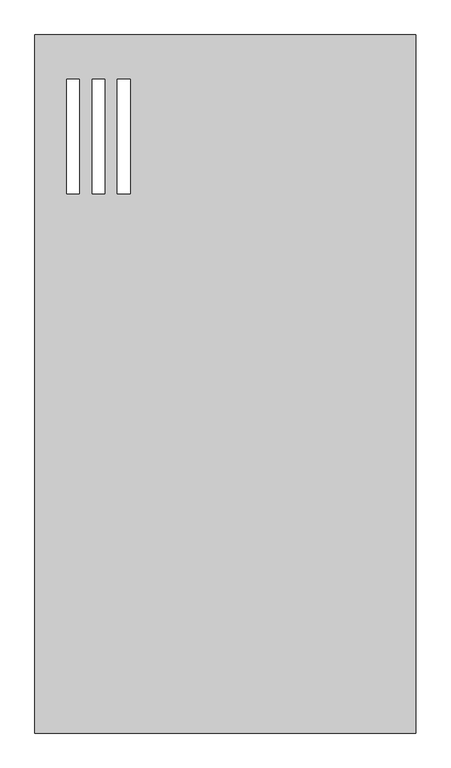
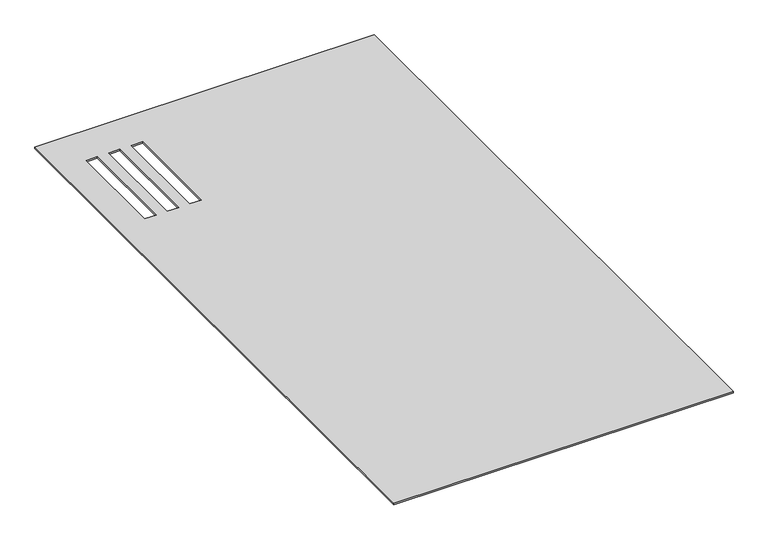
"""IFC4 building model written with IfcOpenShell, lengths in millimetres: proxy geometry, TSP Geyser Electrcical 300L : TSP Geyser Electrcical 300L."""

from ifc_helpers import new_model, si_unit, origin, origin_with_axes, place, context, project, spatial, polyline, outline, extrude, source, transform, mapped, element, save


def electrical_fixtures_aa66fa3b(model_context):
    return source(origin(), model_context, "Body", "SweptSolid", [
        extrude(outline(polyline([(-600.0, 600.0), (0.0, 600.0), (0.0, -500.0), (-600.0, -500.0), (-600.0, 600.0)]), holes=[polyline([(-530.0, 530.0), (-550.0, 530.0), (-550.0, 350.0), (-530.0, 350.0), (-530.0, 530.0)]), polyline([(-490.0, 530.0), (-510.0, 530.0), (-510.0, 350.0), (-490.0, 350.0), (-490.0, 530.0)]), polyline([(-450.0, 530.0), (-470.0, 530.0), (-470.0, 350.0), (-450.0, 350.0), (-450.0, 530.0)])]), origin_with_axes(), (0.0, 0.0, 1.0), 3.0),
    ])


if __name__ == "__main__":
    model = new_model("IFC4")
    model_context = context("Model", 3, world=origin())
    ifc_project = project(units=[si_unit("LENGTHUNIT", "METRE", prefix="MILLI")], contexts=[model_context])
    site = spatial("IfcSite", under=ifc_project)
    building = spatial("IfcBuilding", under=site)
    placement = place(None, origin())
    electrical_fixtures_shape = electrical_fixtures_aa66fa3b(model_context)
    element("IfcBuildingElementProxy", 1, Name="TSP Geyser Electrcical 300L : TSP Geyser Electrcical 300L", ObjectType="TSP Geyser Electrcical 300L : TSP Geyser Electrcical 300L", at=placement, inside=building, context=model_context, shape_type="MappedRepresentation", body=[
        mapped(electrical_fixtures_shape, transform((0.0, 0.0, 0.0), x_axis=(1.0, 0.0, 0.0), y_axis=(0.0, 1.0, 0.0), z_axis=(0.0, 0.0, 1.0))),
    ])
    save(model, "model.ifc")

# Revit data of these elements
# Type "TSP Geyser Electrcical 300L : TSP Geyser Electrcical 300L"
#   Model = "TSP_EGEY300"
#   Default Elevation = 0
# Element 1 (IfcBuildingElementProxy, "TSP Geyser Electrcical 300L : TSP Geyser Electrcical 300L")
#   Materials on its faces: "Aluminum, Anodized Red"
# Materials
#   "Aluminum, Anodized Red": class "Metal", colour RGB 120 120 120, transparency 0, Description = "Anodized aluminum, red", Cost = 0
